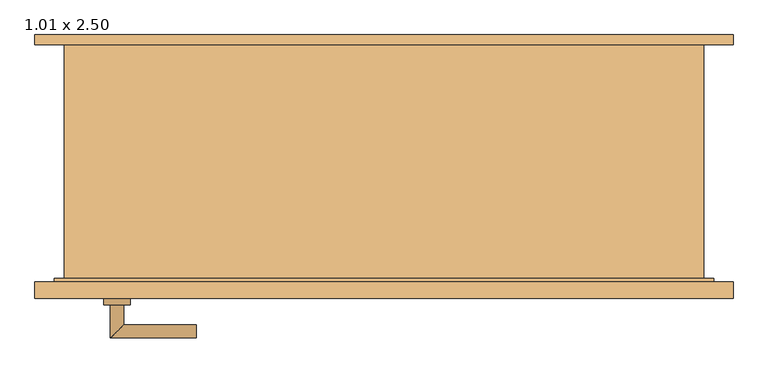
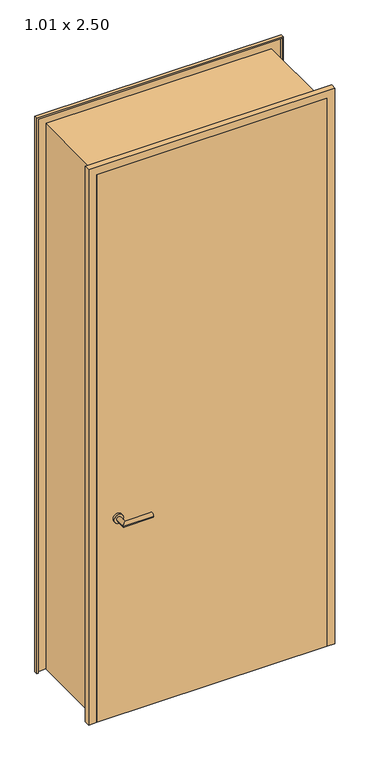
"""IFC4 building model written with IfcOpenShell, lengths in millimetres: door geometry, Drehflügel 1-flg - Stahlzarge : 1.01 x 2.50."""

from ifc_helpers import new_model, si_unit, point, frame, frame_2d, origin, place, context, project, spatial, polyline, circle_curve, ellipse_curve, trimmed, segment, composite_curve, outline, extrude, faceted_brep, source, transform, mapped, element, save
from ifc_brep_helpers import plane_surface, cylinder_surface, advanced_brep


def door_1_01_x_2_50_4be29bae(model_context):
    return source(origin(), model_context, "Body", "SolidModel", [
        advanced_brep(
        [(-415.0, -169.4346141, 1000.0), (-395.0, -169.4346141, 1000.0), (-395.0, -119.4346141, 1000.0), (-415.0, -99.4346141, 1000.0), (-285.0, -99.4346141, 1000.0), (-285.0, -119.4346141, 1000.0)],
        [
            (0, 1, circle_curve(frame((-405.0, -169.4346141, 1000.0), z_axis=(0.0, -1.0, 0.0), x_axis=(1.0, 0.0, 0.0)), 10.0)),
            (1, 0, circle_curve(frame((-405.0, -169.4346141, 1000.0), z_axis=(0.0, -1.0, 0.0), x_axis=(1.0, 0.0, 0.0)), 10.0)),
            (1, 2),
            (2, 3, ellipse_curve(frame((-405.0, -109.4346141, 1000.0), z_axis=(-0.7071067811865385, -0.7071067811865565, 0.0), x_axis=(0.7071067811865563, -0.7071067811865386, 0.0)), 14.1421356, 10.0)),
            (3, 0),
            (3, 2, ellipse_curve(frame((-405.0, -109.4346141, 1000.0), z_axis=(-0.7071067811865385, -0.7071067811865565, 0.0), x_axis=(0.7071067811865563, -0.7071067811865386, 0.0)), 14.1421356, 10.0)),
            (4, 5, circle_curve(frame((-285.0, -109.4346141, 1000.0), z_axis=(1.0, 0.0, 0.0), x_axis=(0.0, -1.0, 0.0)), 10.0)),
            (5, 4, circle_curve(frame((-285.0, -109.4346141, 1000.0), z_axis=(1.0, 0.0, 0.0), x_axis=(0.0, -1.0, 0.0)), 10.0)),
            (2, 5),
            (4, 3),
        ],
        [
            plane_surface(frame((-405.0, -169.4346141, -287.7526403), z_axis=(0.0, -1.0, 0.0), x_axis=(0.0, 0.0, 1.0))),
            cylinder_surface(frame((-405.0, -169.4346141, 1000.0), z_axis=(0.0, -1.0, 0.0), x_axis=(1.0, 0.0, 0.0)), 10.0),
            plane_surface(frame((-285.0, -109.4346141, -287.7526403), z_axis=(1.0, 0.0, 0.0), x_axis=(0.0, 0.0, 1.0))),
            cylinder_surface(frame((-405.0, -109.4346141, 1000.0), z_axis=(-1.0, 0.0, 0.0), x_axis=(0.0, -1.0, 0.0)), 10.0),
        ],
        [
            (0, [[1, 2]]),
            (1, [[3, 4, 5, -2]]),
            (1, [[-5, 6, -3, -1]]),
            (2, [[7, 8]]),
            (3, [[9, -7, 10, -4]]),
            (3, [[-10, -8, -9, -6]]),
        ],
    ),
        advanced_brep(
        [(-395.0, -229.4346141, 1000.0), (-415.0, -229.4346141, 1000.0), (-415.0, -279.4346141, 1000.0), (-395.0, -259.4346141, 1000.0), (-285.0, -259.4346141, 1000.0), (-285.0, -279.4346141, 1000.0)],
        [
            (0, 1, circle_curve(frame((-405.0, -229.4346141, 1000.0), z_axis=(0.0, 1.0, 0.0), x_axis=(-1.0, 0.0, 0.0)), 10.0)),
            (1, 0, circle_curve(frame((-405.0, -229.4346141, 1000.0), z_axis=(0.0, 1.0, 0.0), x_axis=(-1.0, 0.0, 0.0)), 10.0)),
            (1, 2),
            (2, 3, ellipse_curve(frame((-405.0, -269.4346141, 1000.0), z_axis=(-0.7071067811865475, 0.7071067811865475, 0.0), x_axis=(0.7071067811865474, 0.7071067811865476, 0.0)), 14.1421356, 10.0)),
            (3, 0),
            (3, 2, ellipse_curve(frame((-405.0, -269.4346141, 1000.0), z_axis=(-0.7071067811865475, 0.7071067811865475, 0.0), x_axis=(0.7071067811865474, 0.7071067811865476, 0.0)), 14.1421356, 10.0)),
            (4, 5, circle_curve(frame((-285.0, -269.4346141, 1000.0), z_axis=(1.0, 0.0, 0.0), x_axis=(0.0, -1.0, 0.0)), 10.0)),
            (5, 4, circle_curve(frame((-285.0, -269.4346141, 1000.0), z_axis=(1.0, 0.0, 0.0), x_axis=(0.0, -1.0, 0.0)), 10.0)),
            (2, 5),
            (4, 3),
        ],
        [
            plane_surface(frame((-405.0, -229.4346141, -287.7526403), z_axis=(0.0, 1.0, 0.0), x_axis=(0.0, 0.0, 1.0))),
            cylinder_surface(frame((-405.0, -229.4346141, 1000.0), z_axis=(0.0, 1.0, 0.0), x_axis=(-1.0, 0.0, 0.0)), 10.0),
            plane_surface(frame((-285.0, -269.4346141, -287.7526403), z_axis=(1.0, 0.0, 0.0), x_axis=(0.0, 0.0, 1.0))),
            cylinder_surface(frame((-405.0, -269.4346141, 1000.0), z_axis=(-1.0, 0.0, 0.0), x_axis=(0.0, -1.0, 0.0)), 10.0),
        ],
        [
            (0, [[1, 2]]),
            (1, [[3, 4, 5, -2]]),
            (1, [[-5, 6, -3, -1]]),
            (2, [[7, 8]]),
            (3, [[9, -7, 10, -4]]),
            (3, [[-10, -8, -9, -6]]),
        ],
    ),
        extrude(outline(composite_curve([segment(trimmed(circle_curve(frame_2d((1000.0, -405.0)), 20.0), [point((1000.0, -425.0))], [point((1000.0, -385.0))], False, "CARTESIAN"), True, "CONTINUOUS"), segment(trimmed(circle_curve(frame_2d((1000.0, -405.0)), 20.0), [point((1000.0, -385.0))], [point((1000.0, -425.0))], False, "CARTESIAN"), True, "CONTINUOUS")], self_intersect=False)), frame((0.0, -169.4346141, 0.0), z_axis=(0.0, 1.0, 0.0), x_axis=(0.0, 0.0, 1.0)), (0.0, 0.0, 1.0), 10.0),
        extrude(outline(composite_curve([segment(trimmed(circle_curve(frame_2d((1000.0, -405.0)), 20.0), [point((1000.0, -425.0))], [point((1000.0, -385.0))], False, "CARTESIAN"), True, "CONTINUOUS"), segment(trimmed(circle_curve(frame_2d((1000.0, -405.0)), 20.0), [point((1000.0, -385.0))], [point((1000.0, -425.0))], False, "CARTESIAN"), True, "CONTINUOUS")], self_intersect=False)), frame((0.0, -229.4346141, 0.0), z_axis=(0.0, 1.0, 0.0), x_axis=(0.0, 0.0, 1.0)), (0.0, 0.0, 1.0), 10.0),
        extrude(outline(polyline([(495.0, -194.4346141), (495.0, -219.4346141), (-495.0, -219.4346141), (-495.0, -194.4346141), (495.0, -194.4346141)])), frame((0.0, 0.0, 100.0), z_axis=(0.0, 0.0, 1.0), x_axis=(1.0, 0.0, 0.0)), (0.0, 0.0, 1.0), 2490.0),
        faceted_brep([(529.4603207, 180.5653859, 100.0), (529.4603207, 165.5653859, 100.0), (524.4603207, 165.5653859, 100.0), (524.4603207, 175.5653859, 100.0), (485.0, 175.5653859, 100.0), (485.0, -189.4346141, 100.0), (500.0, -189.4346141, 100.0), (500.0, -214.4346141, 100.0), (524.4603207, -214.4346141, 100.0), (524.4603207, -194.4346141, 100.0), (529.4603207, -194.4346141, 100.0), (529.4603207, -219.4346141, 100.0), (495.0, -219.4346141, 100.0), (495.0, -194.4346141, 100.0), (480.0, -194.4346141, 100.0), (480.0, 180.5653859, 100.0), (480.0, 180.5653859, 2575.0), (-480.0, 180.5653859, 2575.0), (-480.0, 180.5653859, 100.0), (-529.4603207, 180.5653859, 100.0), (-529.4603207, 180.5653859, 2624.4603207), (529.4603207, 180.5653859, 2624.4603207), (480.0, -194.4346141, 2575.0), (495.0, -194.4346141, 2590.0), (-495.0, -194.4346141, 2590.0), (-495.0, -194.4346141, 100.0), (-480.0, -194.4346141, 100.0), (-480.0, -194.4346141, 2575.0), (495.0, -219.4346141, 2590.0), (529.4603207, -219.4346141, 2624.4603207), (-529.4603207, -219.4346141, 2624.4603207), (-529.4603207, -219.4346141, 100.0), (-495.0, -219.4346141, 100.0), (-495.0, -219.4346141, 2590.0), (529.4603207, -194.4346141, 2624.4603207), (524.4603207, -194.4346141, 2619.4603207), (-524.4603207, -194.4346141, 2619.4603207), (-524.4603207, -194.4346141, 100.0), (-529.4603207, -194.4346141, 100.0), (-529.4603207, -194.4346141, 2624.4603207), (524.4603207, -214.4346141, 2619.4603207), (500.0, -214.4346141, 2595.0), (-500.0, -214.4346141, 2595.0), (-500.0, -214.4346141, 100.0), (-524.4603207, -214.4346141, 100.0), (-524.4603207, -214.4346141, 2619.4603207), (500.0, -189.4346141, 2595.0), (485.0, -189.4346141, 2580.0), (-485.0, -189.4346141, 2580.0), (-485.0, -189.4346141, 100.0), (-500.0, -189.4346141, 100.0), (-500.0, -189.4346141, 2595.0), (485.0, 175.5653859, 2580.0), (524.4603207, 175.5653859, 2619.4603207), (-524.4603207, 175.5653859, 2619.4603207), (-524.4603207, 175.5653859, 100.0), (-485.0, 175.5653859, 100.0), (-485.0, 175.5653859, 2580.0), (524.4603207, 165.5653859, 2619.4603207), (529.4603207, 165.5653859, 2624.4603207), (-529.4603207, 165.5653859, 2624.4603207), (-529.4603207, 165.5653859, 100.0), (-524.4603207, 165.5653859, 100.0), (-524.4603207, 165.5653859, 2619.4603207)], [[[0, 1, 2, 3, 4, 5, 6, 7, 8, 9, 10, 11, 12, 13, 14, 15]], [[15, 16, 17, 18, 19, 20, 21, 0]], [[14, 22, 16, 15]], [[13, 23, 24, 25, 26, 27, 22, 14]], [[12, 28, 23, 13]], [[11, 29, 30, 31, 32, 33, 28, 12]], [[10, 34, 29, 11]], [[9, 35, 36, 37, 38, 39, 34, 10]], [[8, 40, 35, 9]], [[7, 41, 42, 43, 44, 45, 40, 8]], [[6, 46, 41, 7]], [[5, 47, 48, 49, 50, 51, 46, 6]], [[4, 52, 47, 5]], [[3, 53, 54, 55, 56, 57, 52, 4]], [[2, 58, 53, 3]], [[1, 59, 60, 61, 62, 63, 58, 2]], [[0, 21, 59, 1]], [[20, 19, 61, 60]], [[19, 18, 26, 25, 32, 31, 38, 37, 44, 43, 50, 49, 56, 55, 62, 61]], [[27, 26, 18, 17]], [[33, 32, 25, 24]], [[39, 38, 31, 30]], [[45, 44, 37, 36]], [[51, 50, 43, 42]], [[57, 56, 49, 48]], [[63, 62, 55, 54]], [[22, 27, 17, 16]], [[28, 33, 24, 23]], [[34, 39, 30, 29]], [[40, 45, 36, 35]], [[46, 51, 42, 41]], [[52, 57, 48, 47]], [[58, 63, 54, 53]], [[21, 20, 60, 59]]]),
    ])


if __name__ == "__main__":
    model = new_model("IFC4")
    model_context = context("Model", 3, world=origin())
    ifc_project = project(units=[si_unit("LENGTHUNIT", "METRE", prefix="MILLI")], contexts=[model_context])
    site = spatial("IfcSite", under=ifc_project)
    building = spatial("IfcBuilding", under=site)
    placement = place(None, origin())
    door_1_01_x_2_50_shape = door_1_01_x_2_50_4be29bae(model_context)
    element("IfcDoor", 1, ObjectType="Drehflügel 1-flg - Stahlzarge : 1.01 x 2.50", at=placement, inside=building, context=model_context, shape_type="MappedRepresentation", body=[
        mapped(door_1_01_x_2_50_shape, transform((0.0, 0.0, 0.0), x_axis=(1.0, 0.0, 0.0), y_axis=(0.0, 1.0, 0.0), z_axis=(0.0, 0.0, 1.0))),
    ])
    save(model, "model.ifc")

# Revit data of these elements
# Type "Drehflügel 1-flg - Stahlzarge : 1.01 x 2.50"
#   Type Mark = "29"
#   Operation = "SingleSwingRight"
#   Keynote = "16.03"
#   Analytic Construction = "Metall"
#   Thermal Resistance (R) = 0.270117 (m²·K)/W
#   Heat Transfer Coefficient (U) = 3.7021 W/(m²·K)
#   Rough Width = 1.010 m
#   Rough Height [instance default] = 2.600 m
#   Höhe Türgriff [instance default] = 0.900 m
#   Height = 2.500 m
#   Fußbodenaufbau [instance default] = 0.100 m
#   Width = 1.010 m
#   Sichtbarkeit Sturzlinien [instance default] = yes
#   Türgriff auswählen [instance default] = element 221079
#   Türgriff [instance default] = none
#   Türflügel [instance default] = none
#   Rahmen/Pfosten [instance default] = Metall - Lackiert - Grau
#   Visual Light Transmittance = 0
#   Solar Heat Gain Coefficient = 0
#   Function = (empty or 0)
#   Wall Closure = (empty or 0)
# Element 1 (IfcDoor, "Drehflügel 1-flg - Stahlzarge : 1.01 x 2.50")
#   Materials on its faces: "Metall - Lackiert - Grau", "Metall - Chrom", "Holz - Birke"
# Materials
#   "Metall - Lackiert - Grau": class "Farbe 1", colour RGB 98 98 98, transparency 0, Cost = 0
#   "Metall - Chrom": class "Metall", colour RGB 247 247 247, transparency 0, Cost = 0
#   "Holz - Birke": class "Holz", colour RGB 213 164 103, transparency 0, Cost = 0
